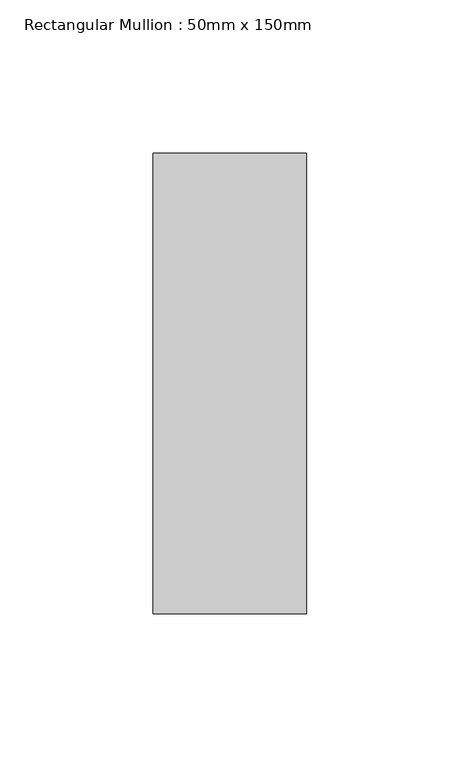
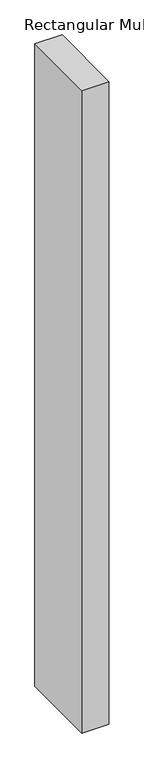
"""IFC4 building model written with IfcOpenShell, lengths in millimetres: member geometry, Rectangular Mullion : 50mm x 150mm."""

from ifc_helpers import new_model, si_unit, frame, origin, place, context, project, spatial, polyline, outline, extrude, source, transform, mapped, element, save


def rectangular_mullion_50mm_x_150mm_46426fc7(model_context):
    return source(origin(), model_context, "Body", "SweptSolid", [
        extrude(outline(polyline([(25.0, 75.0), (25.0, -75.0), (-25.0, -75.0), (-25.0, 75.0), (25.0, 75.0)])), frame((0.0, 0.0, -1253.5714288), z_axis=(0.0, 0.0, 1.0), x_axis=(1.0, 0.0, 0.0)), (0.0, 0.0, 1.0), 1253.5714288),
    ])


if __name__ == "__main__":
    model = new_model("IFC4")
    model_context = context("Model", 3, world=origin())
    ifc_project = project(units=[si_unit("LENGTHUNIT", "METRE", prefix="MILLI")], contexts=[model_context])
    site = spatial("IfcSite", under=ifc_project)
    building = spatial("IfcBuilding", under=site)
    placement = place(None, origin())
    rectangular_mullion_50mm_x_150mm_shape = rectangular_mullion_50mm_x_150mm_46426fc7(model_context)
    element("IfcMember", 1, ObjectType="Rectangular Mullion : 50mm x 150mm", at=placement, inside=building, context=model_context, shape_type="MappedRepresentation", body=[
        mapped(rectangular_mullion_50mm_x_150mm_shape, transform((0.0, 0.0, 0.0), x_axis=(1.0, 0.0, 0.0), y_axis=(0.0, 1.0, 0.0), z_axis=(0.0, 0.0, 1.0))),
    ])
    save(model, "model.ifc")

# Revit data of these elements
# Type "Rectangular Mullion : 50mm x 150mm"
#   built-in parameter 1007304 = 0.492126 (stored number, unit not read)
#   built-in parameter 1007301 = 0.082021 (stored number, unit not read)
#   built-in parameter 1007300 = 0.082021 (stored number, unit not read)
# Element 1 (IfcMember, "Rectangular Mullion : 50mm x 150mm")
#   Materials on its faces: "Aluminum"
# Materials
#   "Aluminum": class "Metal", colour RGB 247 247 247, transparency 0, Description = "Aluminum 6061", Cost = 0
